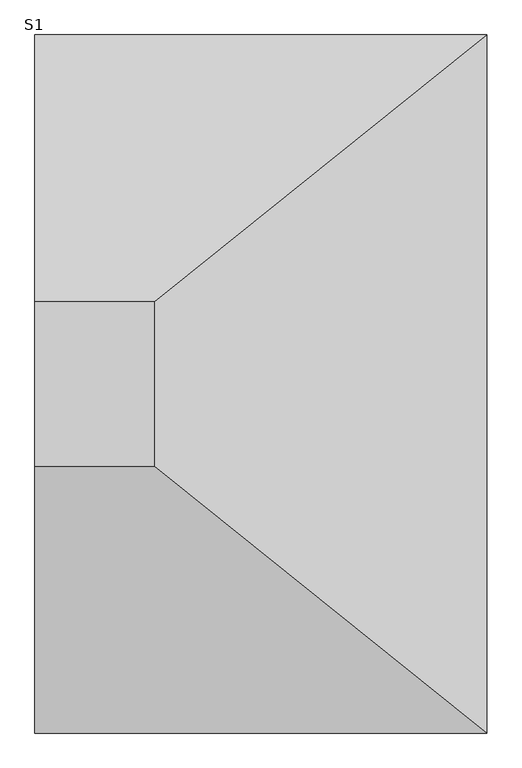
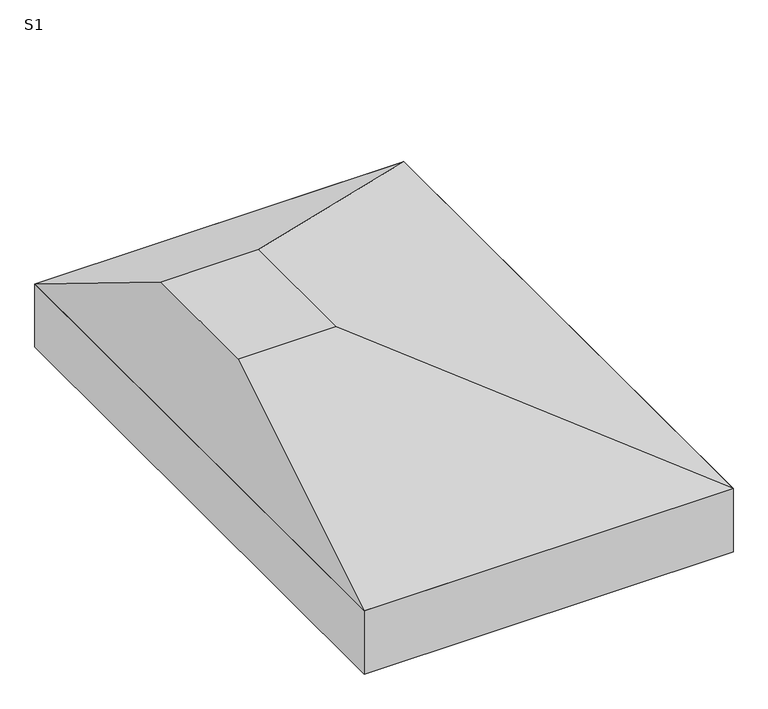
"""IFC4 building model written with IfcOpenShell, lengths in millimetres: fastener geometry, TQS - Sapata : S1."""

from ifc_helpers import new_model, si_unit, frame, origin, place, context, project, spatial, polyline, outline, extrude, faceted_brep, source, transform, mapped, element, save


def s1_ccae0304(model_context):
    return source(origin(), model_context, "Body", "SolidModel", [
        faceted_brep([(-460.0, 0.0, 0.0), (-750.0, 0.0, 0.0), (-750.0, -400.0, 0.0), (-460.0, -400.0, 0.0), (350.0, 650.0, -400.0), (350.0, -1050.0, -400.0), (-750.0, -1050.0, -400.0), (-750.0, 650.0, -400.0)], [[[0, 1, 2, 3]], [[4, 5, 6, 7]], [[4, 7, 1, 0]], [[7, 6, 2, 1]], [[6, 5, 3, 2]], [[5, 4, 0, 3]]]),
        extrude(outline(polyline([(350.0, 650.0), (350.0, -1050.0), (-750.0, -1050.0), (-750.0, 650.0), (350.0, 650.0)])), frame((0.0, 0.0, -600.0), z_axis=(0.0, 0.0, 1.0), x_axis=(1.0, 0.0, 0.0)), (0.0, 0.0, 1.0), 200.0),
    ])


if __name__ == "__main__":
    model = new_model("IFC4")
    model_context = context("Model", 3, world=origin())
    ifc_project = project(units=[si_unit("LENGTHUNIT", "METRE", prefix="MILLI")], contexts=[model_context])
    site = spatial("IfcSite", under=ifc_project)
    building = spatial("IfcBuilding", under=site)
    placement = place(None, origin())
    s1_shape = s1_ccae0304(model_context)
    element("IfcFastener", 1, ObjectType="TQS - Sapata : S1", at=placement, inside=building, context=model_context, shape_type="MappedRepresentation", body=[
        mapped(s1_shape, transform((0.0, 0.0, 0.0), x_axis=(1.0, 0.0, 0.0), y_axis=(0.0, 1.0, 0.0), z_axis=(0.0, 0.0, 1.0))),
    ])
    save(model, "model.ifc")

# Revit data of these elements
# Type "TQS - Sapata : S1"
#   TY = 0.40 m
#   TX = 0.29 m
#   HS = 0.60 m
#   H0 = 0.20 m
#   EXCYABS = 0.85 m
#   EXCY = 0.00 m
#   EXCXABS = 0.145 m
#   EXCX = -0.405 m
#   DIMY = 1.70 m
#   DIMX = 1.10 m
#   Material estrutural = Concreto - Concreto concretado no local
#   Width = 0
#   Length = 0
# Element 1 (IfcFastener, "TQS - Sapata : S1")
#   Materials on its faces: "Concreto - Concreto concretado no local"
# Materials
#   "Concreto - Concreto concretado no local": class "Concreto", colour RGB 192 192 192, transparency 0
